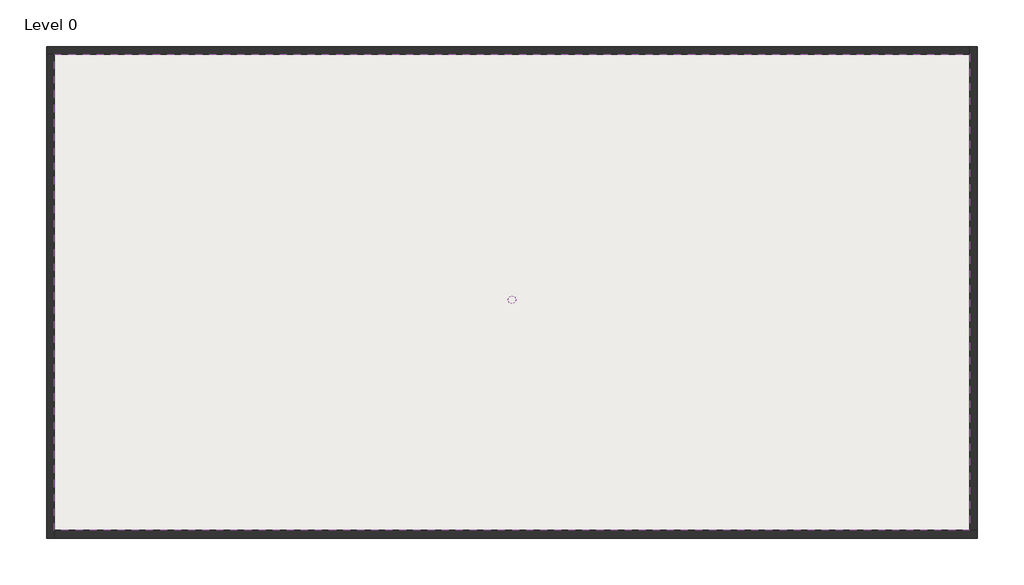
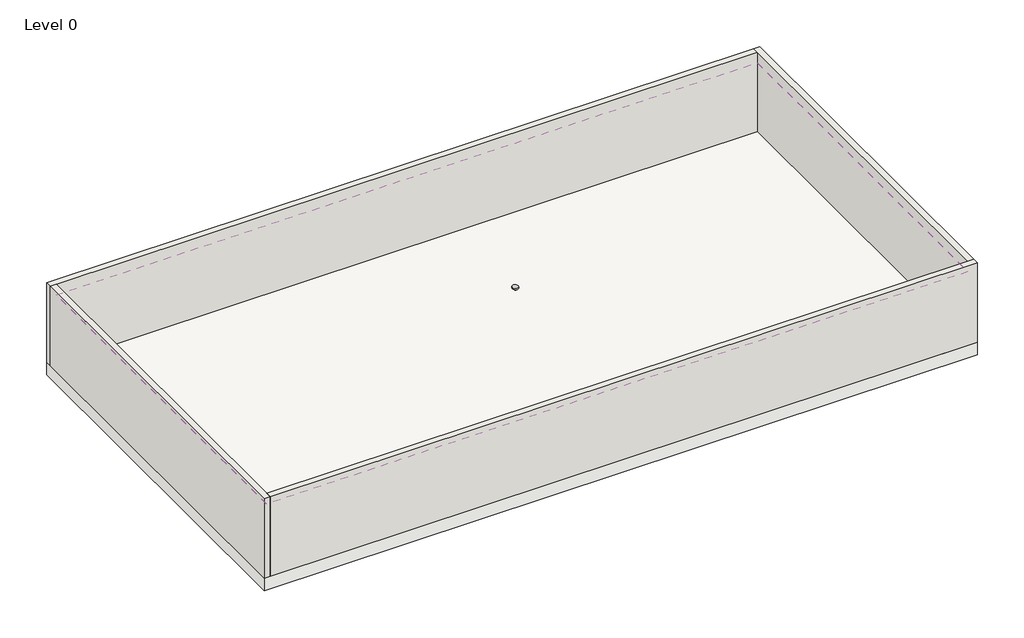
# One storey: 4 walls, 1 covering, 1 electric appliance, 1 slab.
"""IFC4 building model written with IfcOpenShell, lengths in millimetres."""

import ifcopenshell
import ifcopenshell.guid

model = None  # the IFC model being written
_history = None  # IfcOwnerHistory: only IFC2X3 demands one
_inside = {}  # id of a spatial element -> (the spatial element, [elements in it])
_under = {}  # id of a project, library or spatial element -> (it, [spatial elements below it])
_declared = {}  # id of a project -> (the project, [libraries it declares])
_typed = {}  # id of a type object -> (the type object, [elements of that type])
_made_of = {}  # id of a material, layer set ... -> (it, [elements and type objects made of it])


def new_model(schema):
    """Start an empty IFC model of exactly this schema.

    Asked for "IFC4X3", IfcOpenShell would pick the latest addendum, in which some entities
    have other attributes; the version numbers below select the first issue.
    IFC2X3 requires an IfcOwnerHistory on every rooted entity: one is made here for all.
    """
    global model, _history
    if schema == "IFC4X3":
        model = ifcopenshell.file(schema_version=(4, 3, 0, 0))
    else:
        model = ifcopenshell.file(schema=schema)
    _inside.clear()
    _under.clear()
    _declared.clear()
    _typed.clear()
    _made_of.clear()
    _history = None
    if model.schema == "IFC2X3":
        org = make("IfcOrganization", Name="unknown")
        user = make(
            "IfcPersonAndOrganization",
            ThePerson=make("IfcPerson", FamilyName="unknown"),
            TheOrganization=org,
        )
        app = make(
            "IfcApplication",
            ApplicationDeveloper=org,
            Version="unknown",
            ApplicationFullName="unknown",
            ApplicationIdentifier="unknown",
        )
        _history = make(
            "IfcOwnerHistory",
            OwningUser=user,
            OwningApplication=app,
            ChangeAction="ADDED",
            CreationDate=0,
        )
    return model


def make(cls, **values):
    """One entity of the class cls with the attributes given. An attribute that is None is left unset."""
    return model.create_entity(
        cls, **{name: value for name, value in values.items() if value is not None}
    )


def rooted(cls, **values):
    """An entity with a GlobalId (a new one), such as an element, a storey or a relation."""
    return make(cls, GlobalId=ifcopenshell.guid.new(), OwnerHistory=_history, **values)


def si_unit(unit_type, name, prefix=None):
    """IfcSIUnit, for example si_unit("LENGTHUNIT", "METRE", prefix="MILLI")."""
    return make("IfcSIUnit", UnitType=unit_type, Prefix=prefix, Name=name)


def assignment(units):
    """IfcUnitAssignment: the units of a project."""
    return None if units is None else make("IfcUnitAssignment", Units=units)


def point(xyz):
    """IfcCartesianPoint."""
    return None if xyz is None else make("IfcCartesianPoint", Coordinates=xyz)


def direction(xyz):
    """IfcDirection."""
    return None if xyz is None else make("IfcDirection", DirectionRatios=xyz)


def frame(location, z_axis=None, x_axis=None):
    """IfcAxis2Placement3D, a coordinate frame: its origin and axes. An axis left out is left unset."""
    return make(
        "IfcAxis2Placement3D",
        Location=point(location),
        Axis=direction(z_axis),
        RefDirection=direction(x_axis),
    )


def frame_2d(location, x_axis=None):
    """IfcAxis2Placement2D, a coordinate frame in the plane: its origin and x axis."""
    return make(
        "IfcAxis2Placement2D", Location=point(location), RefDirection=direction(x_axis)
    )


def origin():
    """The frame at (0, 0, 0) with its axes left unset."""
    return frame((0.0, 0.0, 0.0))


def origin_with_axes():
    """The frame at (0, 0, 0) with the z axis (0, 0, 1) and the x axis (1, 0, 0) written out."""
    return frame((0.0, 0.0, 0.0), z_axis=(0.0, 0.0, 1.0), x_axis=(1.0, 0.0, 0.0))


def origin_2d():
    """The frame at (0, 0) in the plane with its x axis left unset."""
    return frame_2d((0.0, 0.0))


def place(relative_to, where):
    """IfcLocalPlacement: puts the frame where relative to a parent placement (None: the world)."""
    return make(
        "IfcLocalPlacement", PlacementRelTo=relative_to, RelativePlacement=where
    )


def context(
    kind, dimensions, precision=None, world=None, true_north=None, identifier=None
):
    """IfcGeometricRepresentationContext, for example the 3D "Model" context."""
    return make(
        "IfcGeometricRepresentationContext",
        ContextIdentifier=identifier,
        ContextType=kind,
        CoordinateSpaceDimension=dimensions,
        Precision=precision,
        WorldCoordinateSystem=world,
        TrueNorth=true_north,
    )


def project(units=None, contexts=None):
    """IfcProject with its units and contexts."""
    return rooted(
        "IfcProject",
        Name="project",
        RepresentationContexts=contexts,
        UnitsInContext=assignment(units),
    )


def spatial(cls, under=None, at=None, **own):
    """A site, building, storey or space (cls), placed at a placement, below another one or the project."""
    s = rooted(cls, ObjectPlacement=at, **own)
    if under is not None:
        _under.setdefault(under.id(), (under, []))[1].append(s)
    return s


def polyline(points):
    """IfcPolyline through the points."""
    return make("IfcPolyline", Points=[point(p) for p in points])


def circle_curve(where, radius):
    """IfcCircle in the frame where."""
    return make("IfcCircle", Position=where, Radius=radius)


def trimmed(basis, trim1, trim2, sense, master):
    """IfcTrimmedCurve: the piece of a basis curve between two trims."""
    return make(
        "IfcTrimmedCurve",
        BasisCurve=basis,
        Trim1=trim1,
        Trim2=trim2,
        SenseAgreement=sense,
        MasterRepresentation=master,
    )


def segment(curve, same_sense, transition):
    """IfcCompositeCurveSegment."""
    return make(
        "IfcCompositeCurveSegment",
        Transition=transition,
        SameSense=same_sense,
        ParentCurve=curve,
    )


def composite_curve(segments, self_intersect=None):
    """IfcCompositeCurve: segments joined end to end."""
    return make("IfcCompositeCurve", Segments=segments, SelfIntersect=self_intersect)


def outline(outer, holes=None, kind="AREA"):
    """IfcArbitraryClosedProfileDef: a profile drawn as a closed curve; with holes, ...WithVoids."""
    if holes is None:
        return make("IfcArbitraryClosedProfileDef", ProfileType=kind, OuterCurve=outer)
    return make(
        "IfcArbitraryProfileDefWithVoids",
        ProfileType=kind,
        OuterCurve=outer,
        InnerCurves=holes,
    )


def extrude(swept, where, along, depth):
    """IfcExtrudedAreaSolid: the profile swept, set in the frame where, extruded along a direction by depth."""
    return make(
        "IfcExtrudedAreaSolid",
        SweptArea=swept,
        Position=where,
        ExtrudedDirection=direction(along),
        Depth=depth,
    )


def faces_of(points, faces, orient=None, outer=None):
    """IfcFace entities. A face is a list of loops; a loop is a list of indices into points, from 0.

    orient and outer hold one flag for each loop. By default every Orientation is true, the
    first loop of a face is its IfcFaceOuterBound and the others are IfcFaceBound.
    """
    made = []
    for i, loops in enumerate(faces):
        bounds = []
        for j, loop in enumerate(loops):
            is_outer = j == 0 if outer is None else outer[i][j]
            bounds.append(
                make(
                    "IfcFaceOuterBound" if is_outer else "IfcFaceBound",
                    Bound=make("IfcPolyLoop", Polygon=[points[k] for k in loop]),
                    Orientation=True if orient is None else orient[i][j],
                )
            )
        made.append(make("IfcFace", Bounds=bounds))
    return made


def faceted_brep(points, faces, orient=None, outer=None, voids=None):
    """IfcFacetedBrep: a solid bounded by flat faces; with voids (closed shells), ...WithVoids."""
    shared = [point(p) for p in points]
    hull = make("IfcClosedShell", CfsFaces=faces_of(shared, faces, orient, outer))
    if voids is None:
        return make("IfcFacetedBrep", Outer=hull)
    return make(
        "IfcFacetedBrepWithVoids",
        Outer=hull,
        Voids=[
            make(cls, CfsFaces=faces_of(shared, fs, o, b)) for cls, fs, o, b in voids
        ],
    )


def shape(context_of_items, identifier, shape_type, items):
    """IfcShapeRepresentation: the items that make up one representation, for example the "Body"."""
    return make(
        "IfcShapeRepresentation",
        ContextOfItems=context_of_items,
        RepresentationIdentifier=identifier,
        RepresentationType=shape_type,
        Items=items,
    )


def source(mapping_origin, context_of_items, identifier, shape_type, items):
    """IfcRepresentationMap: a shape defined once, which mapped items show again and again."""
    return make(
        "IfcRepresentationMap",
        MappingOrigin=mapping_origin,
        MappedRepresentation=shape(context_of_items, identifier, shape_type, items),
    )


def transform(
    local_origin,
    x_axis=None,
    y_axis=None,
    z_axis=None,
    scale=None,
    scale2=None,
    scale3=None,
    uniform=True,
):
    """IfcCartesianTransformationOperator3D, or its non-uniform kind. x_axis, y_axis, z_axis: its Axis1, 2, 3."""
    if uniform:
        return make(
            "IfcCartesianTransformationOperator3D",
            Axis1=direction(x_axis),
            Axis2=direction(y_axis),
            LocalOrigin=point(local_origin),
            Scale=scale,
            Axis3=direction(z_axis),
        )
    return make(
        "IfcCartesianTransformationOperator3DnonUniform",
        Axis1=direction(x_axis),
        Axis2=direction(y_axis),
        LocalOrigin=point(local_origin),
        Scale=scale,
        Axis3=direction(z_axis),
        Scale2=scale2,
        Scale3=scale3,
    )


def mapped(mapping_source, mapping_target):
    """IfcMappedItem: shows the shape of a source again, moved by a transform."""
    return make(
        "IfcMappedItem", MappingSource=mapping_source, MappingTarget=mapping_target
    )


def made_of(thing, what):
    """Note that an element or type object is made of a material, layer set ...; save() writes the relation."""
    if what is not None:
        _made_of.setdefault(what.id(), (what, []))[1].append(thing)
    return thing


def element(
    cls,
    number,
    at=None,
    inside=None,
    cuts=None,
    type_object=None,
    material=None,
    context=None,
    identifier="Body",
    shape_type=None,
    held_by="IfcProductDefinitionShape",
    body=None,
    shapes=None,
    **own,
):
    """One element of the class cls, such as IfcWall. Its Tag is "e" and its number.

    at: its placement. inside: the storey or other place that contains it. cuts: it is an
    opening in that element (IfcRelVoidsElement). A single representation is given by context,
    identifier, shape_type and body (its items); several are given by shapes. held_by: the class
    of the entity that holds the representations. save() writes the other relations.
    """
    e = rooted(cls, Tag="e%d" % number, ObjectPlacement=at, **own)
    if body is not None:
        shapes = [shape(context, identifier, shape_type, body)]
    if shapes is not None:
        e.Representation = make(held_by, Representations=shapes)
    if inside is not None:
        _inside.setdefault(inside.id(), (inside, []))[1].append(e)
    if cuts is not None:
        rooted(
            "IfcRelVoidsElement", RelatingBuildingElement=cuts, RelatedOpeningElement=e
        )
    if type_object is not None:
        _typed.setdefault(type_object.id(), (type_object, []))[1].append(e)
    return made_of(e, material)


def aggregate(whole, parts):
    """IfcRelAggregates: a whole, such as a stair, and the parts it consists of."""
    return rooted("IfcRelAggregates", RelatingObject=whole, RelatedObjects=parts)


def save(model, path):
    """Write the relations noted so far, then the file.

    IfcRelAggregates (storeys below a building ...), IfcRelContainedInSpatialStructure (elements
    in a storey), IfcRelDefinesByType, IfcRelAssociatesMaterial and IfcRelDeclares: one each for
    every whole, place, type object, material and project.
    """
    for whole, parts in _under.values():
        aggregate(whole, parts)
    for where, things in _inside.values():
        rooted(
            "IfcRelContainedInSpatialStructure",
            RelatedElements=things,
            RelatingStructure=where,
        )
    for kind, things in _typed.values():
        rooted("IfcRelDefinesByType", RelatedObjects=things, RelatingType=kind)
    for what, things in _made_of.values():
        rooted("IfcRelAssociatesMaterial", RelatedObjects=things, RelatingMaterial=what)
    for by, libraries in _declared.values():
        rooted("IfcRelDeclares", RelatingContext=by, RelatedDefinitions=libraries)
    model.write(path)


def electric_appliance_a5c8b711(model_context):
    return source(origin(), model_context, "Body", "SweptSolid", [
        extrude(outline(composite_curve([segment(trimmed(circle_curve(origin_2d(), 10.0), [point((-10.0, 0.0))], [point((10.0, 0.0))], False, "CARTESIAN"), True, "CONTINUOUS"), segment(trimmed(circle_curve(origin_2d(), 10.0), [point((10.0, 0.0))], [point((-10.0, 0.0))], False, "CARTESIAN"), True, "CONTINUOUS")], self_intersect=False)), frame((0.0, 0.0, 50.0), z_axis=(0.0, 0.0, 1.0), x_axis=(1.0, 0.0, 0.0)), (0.0, 0.0, 1.0), 81.4052538),
        extrude(outline(composite_curve([segment(trimmed(circle_curve(origin_2d(), 110.0), [point((-110.0, 0.0))], [point((110.0, 0.0))], False, "CARTESIAN"), True, "CONTINUOUS"), segment(trimmed(circle_curve(origin_2d(), 110.0), [point((110.0, 0.0))], [point((-110.0, 0.0))], False, "CARTESIAN"), True, "CONTINUOUS")], self_intersect=False)), origin_with_axes(), (0.0, 0.0, 1.0), 50.0),
    ])


model = new_model("IFC4")

# Units and contexts
model_context = context("Model", 3, world=origin())
ifc_project = project(units=[si_unit("LENGTHUNIT", "METRE", prefix="MILLI")], contexts=[model_context])

# Site, building, storey
site = spatial("IfcSite", under=ifc_project)
building = spatial("IfcBuilding", under=site)
storey = spatial("IfcBuildingStorey", under=building, Name="Level 0", Elevation=0.0)

# Covering
placement = place(None, origin())
element("IfcCovering", 1, ObjectType="Plain", at=placement, inside=storey, context=model_context, shape_type="SweptSolid", body=[
    extrude(outline(polyline([(-6728.9458796, 5967.5463282), (18271.0541204, 5967.5463282), (18271.0541204, -7032.4536718), (-6728.9458796, -7032.4536718), (-6728.9458796, 5967.5463282)])), frame((0.0, 0.0, 2600.0), z_axis=(0.0, 0.0, 1.0), x_axis=(1.0, 0.0, 0.0)), (0.0, 0.0, 1.0), 57.0),
])

# Electric appliance
electric_appliance_shape = electric_appliance_a5c8b711(model_context)
element("IfcElectricAppliance", 2, ObjectType="Wifi Access Point : Wifi Access Point", at=placement, inside=storey, context=model_context, shape_type="MappedRepresentation", body=[
    mapped(electric_appliance_shape, transform((5771.0541204, -732.4536718, 2600.0), x_axis=(1.0, 0.0, 0.0), y_axis=(0.0, -1.0, 0.0), z_axis=(0.0, 0.0, -1.0))),
])

# Slab
element("IfcSlab", 3, ObjectType="Floor-Grnd-Susp_65Scr-80Ins-100Blk-75PC", at=placement, inside=storey, context=model_context, shape_type="SweptSolid", body=[
    extrude(outline(polyline([(18486.0541204, 6182.5463282), (18486.0541204, -7247.4536718), (-6943.9458796, -7247.4536718), (-6943.9458796, 6182.5463282), (18486.0541204, 6182.5463282)])), frame((0.0, 0.0, -470.0), z_axis=(0.0, 0.0, 1.0), x_axis=(1.0, 0.0, 0.0)), (0.0, 0.0, 1.0), 470.0),
])

# Walls
element("IfcWall", 4, ObjectType="Wall-Ext_215Bwk", at=placement, inside=storey, context=model_context, shape_type="Brep", body=[
    faceted_brep([(-6943.9458796, 5967.5463282, 0.0), (-6728.9458796, 5967.5463282, 0.0), (18271.0541204, 5967.5463282, 0.0), (18271.0541204, 5967.5463282, 3000.0), (-6728.9458796, 5967.5463282, 3000.0), (-6943.9458796, 5967.5463282, 3000.0), (-6943.9458796, 6182.5463282, 0.0), (-6943.9458796, 6182.5463282, 3000.0), (18271.0541204, 6182.5463282, 3000.0), (18271.0541204, 6182.5463282, 0.0)], [[[0, 1, 2, 3, 4, 5]], [[6, 7, 8, 9]], [[2, 1, 0, 6, 9]], [[5, 4, 3, 8, 7]], [[0, 5, 7, 6]], [[3, 2, 9, 8]]]),
])
element("IfcWall", 5, ObjectType="Wall-Ext_215Bwk", at=placement, inside=storey, context=model_context, shape_type="Brep", body=[
    faceted_brep([(-6728.9458796, -7247.4536718, 0.0), (-6728.9458796, -7032.4536718, 0.0), (-6728.9458796, 5967.5463282, 0.0), (-6728.9458796, 5967.5463282, 3000.0), (-6728.9458796, -7032.4536718, 3000.0), (-6728.9458796, -7247.4536718, 3000.0), (-6943.9458796, -7247.4536718, 0.0), (-6943.9458796, -7247.4536718, 3000.0), (-6943.9458796, 5967.5463282, 3000.0), (-6943.9458796, 5967.5463282, 0.0)], [[[0, 1, 2, 3, 4, 5]], [[6, 7, 8, 9]], [[2, 1, 0, 6, 9]], [[5, 4, 3, 8, 7]], [[0, 5, 7, 6]], [[3, 2, 9, 8]]]),
])
element("IfcWall", 6, ObjectType="Wall-Ext_215Bwk", at=placement, inside=storey, context=model_context, shape_type="Brep", body=[
    faceted_brep([(18486.0541204, -7032.4536718, 0.0), (18271.0541204, -7032.4536718, 0.0), (-6728.9458796, -7032.4536718, 0.0), (-6728.9458796, -7032.4536718, 3000.0), (18271.0541204, -7032.4536718, 3000.0), (18486.0541204, -7032.4536718, 3000.0), (18486.0541204, -7247.4536718, 0.0), (18486.0541204, -7247.4536718, 3000.0), (-6728.9458796, -7247.4536718, 3000.0), (-6728.9458796, -7247.4536718, 0.0)], [[[0, 1, 2, 3, 4, 5]], [[6, 7, 8, 9]], [[2, 1, 0, 6, 9]], [[5, 4, 3, 8, 7]], [[0, 5, 7, 6]], [[3, 2, 9, 8]]]),
])
element("IfcWall", 7, ObjectType="Wall-Ext_215Bwk", at=placement, inside=storey, context=model_context, shape_type="Brep", body=[
    faceted_brep([(18271.0541204, 6182.5463282, 0.0), (18271.0541204, 5967.5463282, 0.0), (18271.0541204, -7032.4536718, 0.0), (18271.0541204, -7032.4536718, 3000.0), (18271.0541204, 5967.5463282, 3000.0), (18271.0541204, 6182.5463282, 3000.0), (18486.0541204, 6182.5463282, 0.0), (18486.0541204, 6182.5463282, 3000.0), (18486.0541204, -7032.4536718, 3000.0), (18486.0541204, -7032.4536718, 0.0)], [[[0, 1, 2, 3, 4, 5]], [[6, 7, 8, 9]], [[2, 1, 0, 6, 9]], [[5, 4, 3, 8, 7]], [[0, 5, 7, 6]], [[3, 2, 9, 8]]]),
])

save(model, "model.ifc")

# Revit data of these elements
# Project information
#   Project Issue Date = "Issue Date"
#   Project Status = "Project Status"
#   Client Name = "Owner"
#   Project Address = "Enter address here"
#   Project Name = "Project Name"
#   Project Number = "Project Number"
# Type "Plain"
#   Keynote = "K40"
#   built-in parameter 1002203 = 1 (stored number, unit not read)
#   built-in parameter 1002202 = 1 (stored number, unit not read)
#   Layers, outside or top first: 0.045 m "Metal Stud Layer" (function 1); 0.012 m "Gypsum Wall Board" (function 1)
# Type "Wifi Access Point : Wifi Access Point"
#   Default Elevation = 1.2 m
# Type "Floor-Grnd-Susp_65Scr-80Ins-100Blk-75PC"
#   Keynote = "E60/130"
#   Function = 0
#   Layers, outside or top first: 0.065 m "Concrete, Sand/Cement Screed" (function 4); 0 m "Vapor Retarder" (function 100); 0.08 m "Rigid insulation" (function 3); 0.15 m "Air" (function 3); 0 m "Damp-proofing" (function 100); 0.1 m "Concrete Masonry, Floor Block" (function 1); 0.075 m "Concrete, Precast" (function 1)
# Type "Wall-Ext_215Bwk"
#   Keynote = "F10"
#   Layers, outside or top first: 0.215 m "Brick, Common" (function 1)
# Element 1 (IfcCovering, "Plain")
#   Height Offset From Level = 2.6 m
#   Phase Created = New Construction
#   Materials on its faces: "Gypsum Wall Board", "Metal Stud Layer"
# Element 2 (IfcElectricAppliance, "Wifi Access Point : Wifi Access Point")
#   Mark = "1"
#   Phase Created = New Construction
# Element 3 (IfcSlab, "Floor-Grnd-Susp_65Scr-80Ins-100Blk-75PC")
#   Height Offset From Level = 0 m
#   Phase Created = New Construction
#   Materials on its faces: "Concrete, Precast", "Concrete, Sand/Cement Screed"
# Elements 4, 5, 6, 7 (IfcWall, "Wall-Ext_215Bwk")
#   Top Offset = 0 m
#   Base Offset = 0 m
#   Unconnected Height = 3 m
#   wall height = 3 m
#   Phase Created = New Construction
#   Base Constraint = Level 0
#   Materials on its faces: "Brick, Common"
# Materials
#   "Metal Stud Layer": class "Metal", colour RGB 127 127 127, transparency 0, Description = "Light gauge steel framing, thermal air layer", Cost = 0
#   "Gypsum Wall Board": class "Generic", colour RGB 249 249 249, transparency 0, Description = "Gypsum Wall Board", Cost = 0
#   "Concrete, Sand/Cement Screed": class "Concrete", colour RGB 127 127 127, transparency 0, Description = "Concrete slab topping", Cost = 0
#   "Vapor Retarder": class "Generic", colour RGB 120 120 120, transparency 0, Description = "Polyethylene film membrane", Cost = 0
#   "Rigid insulation": class "Generic", colour RGB 127 127 127, transparency 0, Description = "Rigid foam insulation board", Cost = 0
#   "Air": class "Gas", colour RGB 255 255 255, transparency 0, Description = "Air", Cost = 0
#   "Damp-proofing": class "Generic", colour RGB 127 127 127, transparency 0, Description = "Damp-proofing", Cost = 0
#   "Concrete Masonry, Floor Block": class "Concrete", colour RGB 181 181 181, transparency 0, Description = "physical material", Cost = 0
#   "Concrete, Precast": class "Concrete", colour RGB 192 192 192, transparency 0, Description = "Precast concrete", Cost = 0
#   "Brick, Common": class "Masonry", colour RGB 170 100 105, transparency 0, Description = "Common brick", Cost = 0
